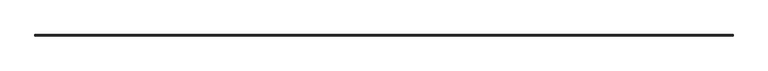
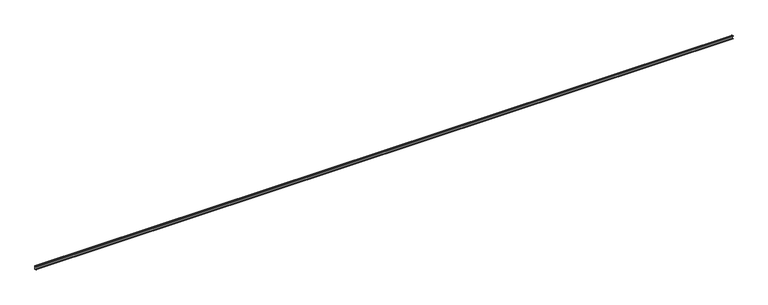
"""IFC4 building model written with IfcOpenShell, lengths in millimetres: beam geometry, 0912_Steel Framing_LC_KDS3530 : H_SB_AR_B03_LC-200x75x25x3.2."""

from ifc_helpers import new_model, si_unit, point, frame, frame_2d, origin, place, context, project, spatial, polyline, circle_curve, trimmed, segment, composite_curve, outline, extrude, source, transform, mapped, element, save


def beam_4465a557(model_context):
    return source(origin(), model_context, "Body", "SweptSolid", [
        extrude(outline(composite_curve([segment(polyline([(18.6, 87.5), (18.6, -87.5)]), True, "CONTINUOUS"), segment(trimmed(circle_curve(frame_2d((6.1, -87.5)), 12.5), [point((18.6, -87.5))], [point((6.1, -100.0))], False, "CARTESIAN"), True, "CONTINUOUS"), segment(polyline([(6.1, -100.0), (-43.9, -100.0)]), True, "CONTINUOUS"), segment(trimmed(circle_curve(frame_2d((-43.9, -87.5)), 12.5), [point((-43.9, -100.0))], [point((-56.4, -87.5))], False, "CARTESIAN"), True, "CONTINUOUS"), segment(polyline([(-56.4, -87.5), (-56.4, -75.0), (-51.9, -75.0), (-51.9, -87.5)]), True, "CONTINUOUS"), segment(trimmed(circle_curve(frame_2d((-43.9, -87.5)), 8.0), [point((-51.9, -87.5))], [point((-43.9, -95.5))], True, "CARTESIAN"), True, "CONTINUOUS"), segment(polyline([(-43.9, -95.5), (6.1, -95.5)]), True, "CONTINUOUS"), segment(trimmed(circle_curve(frame_2d((6.1, -87.5)), 8.0), [point((6.1, -95.5))], [point((14.1, -87.5))], True, "CARTESIAN"), True, "CONTINUOUS"), segment(polyline([(14.1, -87.5), (14.1, 87.5)]), True, "CONTINUOUS"), segment(trimmed(circle_curve(frame_2d((6.1, 87.5)), 8.0), [point((14.1, 87.5))], [point((6.1, 95.5))], True, "CARTESIAN"), True, "CONTINUOUS"), segment(polyline([(6.1, 95.5), (-41.1, 95.5)]), True, "CONTINUOUS"), segment(trimmed(circle_curve(frame_2d((-41.1, 87.5)), 8.0), [point((-41.1, 95.5))], [point((-49.1, 87.5))], True, "CARTESIAN"), True, "CONTINUOUS"), segment(polyline([(-49.1, 87.5), (-49.1, 75.0), (-53.6, 75.0), (-53.6, 87.5)]), True, "CONTINUOUS"), segment(trimmed(circle_curve(frame_2d((-41.1, 87.5)), 12.5), [point((-53.6, 87.5))], [point((-41.1, 100.0))], False, "CARTESIAN"), True, "CONTINUOUS"), segment(polyline([(-41.1, 100.0), (6.1, 100.0)]), True, "CONTINUOUS"), segment(trimmed(circle_curve(frame_2d((6.1, 87.5)), 12.5), [point((6.1, 100.0))], [point((18.6, 87.5))], False, "CARTESIAN"), True, "CONTINUOUS")], self_intersect=False)), frame((-19500.0, 0.0, 0.0), z_axis=(1.0, 0.0, 0.0), x_axis=(0.0, 1.0, 0.0)), (0.0, 0.0, 1.0), 39450.0),
    ])


if __name__ == "__main__":
    model = new_model("IFC4")
    model_context = context("Model", 3, world=origin())
    ifc_project = project(units=[si_unit("LENGTHUNIT", "METRE", prefix="MILLI")], contexts=[model_context])
    site = spatial("IfcSite", under=ifc_project)
    building = spatial("IfcBuilding", under=site)
    placement = place(None, origin())
    beam_shape = beam_4465a557(model_context)
    element("IfcBeam", 1, ObjectType="0912_Steel Framing_LC_KDS3530 : H_SB_AR_B03_LC-200x75x25x3.2", at=placement, inside=building, context=model_context, shape_type="MappedRepresentation", body=[
        mapped(beam_shape, transform((0.0, 0.0, 0.0), x_axis=(1.0, 0.0, 0.0), y_axis=(0.0, 1.0, 0.0), z_axis=(0.0, 0.0, 1.0))),
    ])
    save(model, "model.ifc")

# Revit data of these elements
# Type "0912_Steel Framing_LC_KDS3530 : H_SB_AR_B03_LC-200x75x25x3.2"
#   r = 8 mm
#   d = 25 mm
#   R = 11.2 mm
#   Perimeter = 0.78 m²/m
#   Nominal Weight = 14.00 kgf/m
#   Length [instance default] = 1000 mm
#   B = 75 mm
#   H = 200 mm
#   tw = 3.2 mm
#   x = 18.6 mm
#   A = 1.00 m²
#   Structural Material [instance default] = Steel, 45-345
#   Assembly Code = ""
# Element 1 (IfcBeam, "0912_Steel Framing_LC_KDS3530 : H_SB_AR_B03_LC-200x75x25x3.2")
#   Materials on its faces: "Steel, 45-345"
# Materials
#   "Steel, 45-345": class "Metal", colour RGB 189 187 185, transparency 0, Description = "Steel 345 MPa", Cost = 0
